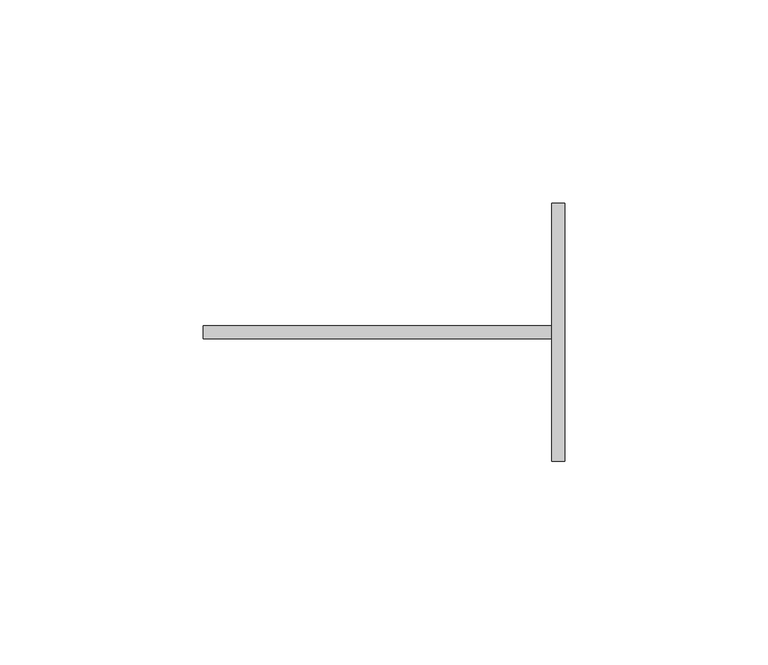
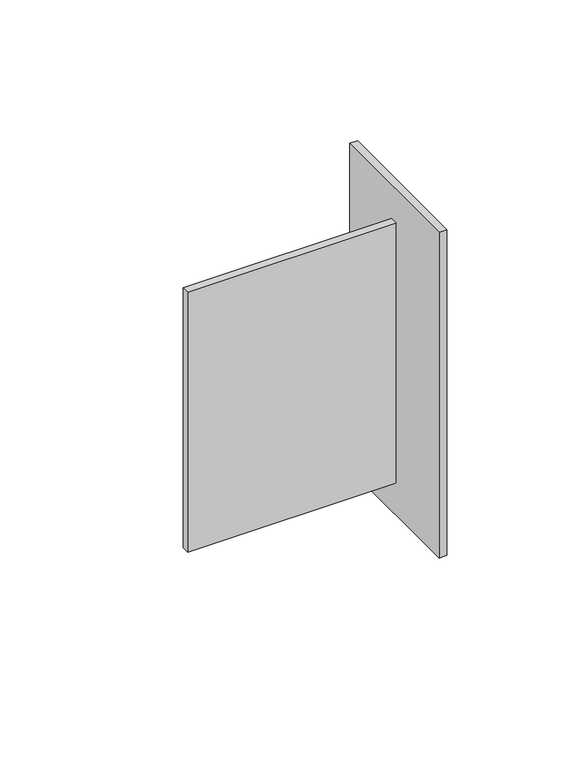
"""IFC4 building model written with IfcOpenShell, lengths in millimetres: proxy geometry, 060523 - W_P_C - Fastenings - Concealed Joist Ties:060523 - W_P_C - Fastenings - Concealed Joist Ties:152590 : 060523 - W_P_C - Fastenings - Concealed Joist Ties:060523 - W_P_C - Fastenings - Concealed Joist Ties:152590."""

from ifc_helpers import new_model, si_unit, frame, origin, place, context, project, spatial, polyline, outline, extrude, source, transform, mapped, element, save


def generic_models_2e03a63b(model_context):
    return source(origin(), model_context, "Body", "SweptSolid", [
        extrude(outline(polyline([(-8392.0465102, 679.071923), (-8392.0465102, 742.571923), (-8388.8715102, 742.571923), (-8388.8715102, 679.071923), (-8392.0465102, 679.071923)])), frame((0.0, 0.0, 3169.0018876), z_axis=(0.0, 0.0, 1.0), x_axis=(1.0, 0.0, 0.0)), (0.0, 0.0, 1.0), 141.2875),
        extrude(outline(polyline([(-8477.7715102, 709.234423), (-8477.7715102, 712.409423), (-8392.0465102, 712.409423), (-8392.0465102, 709.234423), (-8477.7715102, 709.234423)])), frame((0.0, 0.0, 3183.2893876), z_axis=(0.0, 0.0, 1.0), x_axis=(1.0, 0.0, 0.0)), (0.0, 0.0, 1.0), 112.7125),
    ])


if __name__ == "__main__":
    model = new_model("IFC4")
    model_context = context("Model", 3, world=origin())
    ifc_project = project(units=[si_unit("LENGTHUNIT", "METRE", prefix="MILLI")], contexts=[model_context])
    site = spatial("IfcSite", under=ifc_project)
    building = spatial("IfcBuilding", under=site)
    placement = place(None, origin())
    generic_models_shape = generic_models_2e03a63b(model_context)
    element("IfcBuildingElementProxy", 1, Name="060523 - W_P_C - Fastenings - Concealed Joist Ties:060523 - W_P_C - Fastenings - Concealed Joist Ties:152590 : 060523 - W_P_C - Fastenings - Concealed Joist Ties:060523 - W_P_C - Fastenings - Concealed Joist Ties:152590", ObjectType="060523 - W_P_C - Fastenings - Concealed Joist Ties:060523 - W_P_C - Fastenings - Concealed Joist Ties:152590 : 060523 - W_P_C - Fastenings - Concealed Joist Ties:060523 - W_P_C - Fastenings - Concealed Joist Ties:152590", at=placement, inside=building, context=model_context, shape_type="MappedRepresentation", body=[
        mapped(generic_models_shape, transform((0.0, 0.0, 0.0), x_axis=(1.0, 0.0, 0.0), y_axis=(0.0, 1.0, 0.0), z_axis=(0.0, 0.0, 1.0))),
    ])
    save(model, "model.ifc")

# Revit data of these elements
# Type "060523 - W_P_C - Fastenings - Concealed Joist Ties:060523 - W_P_C - Fastenings - Concealed Joist Ties:152590 : 060523 - W_P_C - Fastenings - Concealed Joist Ties:060523 - W_P_C - Fastenings - Concealed Joist Ties:152590"
#   NameOverride = "060523 - W_P_C - Fastenings - Concealed Joist Ties:060523 - W_P_C - Fastenings - Concealed Joist Ties:152590"
#   ObjectTypeOverride = "060523 - W_P_C - Fastenings - Concealed Joist Ties:060523 - W_P_C - Fastenings - Concealed Joist Ties"
#   Reference = "060523 - W_P_C - Fastenings - Concealed Joist Ties"
#   Category = "Generic Models"
#   Tag = "152590"
# Element 1 (IfcBuildingElementProxy, "060523 - W_P_C - Fastenings - Concealed Joist Ties:060523 - W_P_C - Fastenings - Concealed Joist Ties:152590 : 060523 - W_P_C - Fastenings - Concealed Joist Ties:060523 - W_P_C - Fastenings - Concealed Joist Ties:152590")
#   Materials on its faces: "_BEAM HANGER (SEE STRUCT. DWGS) 6017"
# Materials
#   "_BEAM HANGER (SEE STRUCT. DWGS) 6017": class "Unassigned", colour RGB 191 191 191, transparency 0
